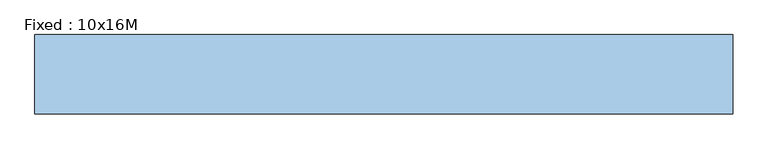
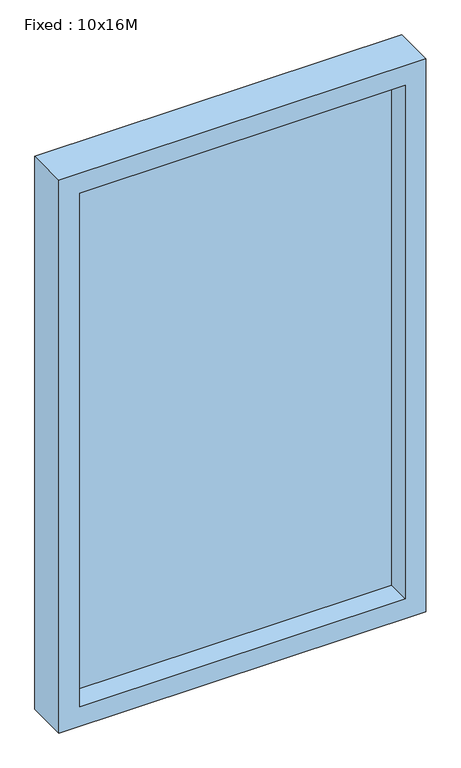
"""IFC4 building model written with IfcOpenShell, lengths in millimetres: window geometry, Fixed : 10x16M."""

from ifc_helpers import new_model, si_unit, frame, origin, place, context, project, spatial, polyline, outline, extrude, source, transform, mapped, element, save


def fixed_10x16m_885135a8(model_context):
    return source(origin(), model_context, "Body", "SweptSolid", [
        extrude(outline(polyline([(2412.0, 506.0), (2412.0, -506.0), (800.0, -506.0), (800.0, 506.0), (2412.0, 506.0)]), holes=[polyline([(857.0, 449.0), (857.0, -449.0), (2355.0, -449.0), (2355.0, 449.0), (857.0, 449.0)])]), frame((0.0, 69.0, 0.0), z_axis=(0.0, 1.0, 0.0), x_axis=(0.0, 0.0, 1.0)), (0.0, 0.0, 1.0), 115.0),
        extrude(outline(polyline([(-449.0, 162.0), (449.0, 162.0), (449.0, 134.0), (-449.0, 134.0), (-449.0, 162.0)])), frame((0.0, 0.0, 857.0), z_axis=(0.0, 0.0, 1.0), x_axis=(1.0, 0.0, 0.0)), (0.0, 0.0, 1.0), 1498.0),
    ])


if __name__ == "__main__":
    model = new_model("IFC4")
    model_context = context("Model", 3, world=origin())
    ifc_project = project(units=[si_unit("LENGTHUNIT", "METRE", prefix="MILLI")], contexts=[model_context])
    site = spatial("IfcSite", under=ifc_project)
    building = spatial("IfcBuilding", under=site)
    placement = place(None, origin())
    fixed_10x16m_shape = fixed_10x16m_885135a8(model_context)
    element("IfcWindow", 1, ObjectType="Fixed : 10x16M", at=placement, inside=building, context=model_context, shape_type="MappedRepresentation", body=[
        mapped(fixed_10x16m_shape, transform((0.0, 0.0, 0.0), x_axis=(1.0, 0.0, 0.0), y_axis=(0.0, 1.0, 0.0), z_axis=(0.0, 0.0, 1.0))),
    ])
    save(model, "model.ifc")

# Revit data of these elements
# Type "Fixed : 10x16M"
#   Type Mark = "59"
#   Creator Organization [instance default] = "© Danish Educational Content"
#   Creator Name [instance default] = "© Erik Falck Jørgensen"
#   Creator Build [instance default] = "2017.0801.0"
#   Analytic Construction = "<None>"
#   length#5 = -22 mm
#   length#4 = -50 mm
#   length#3 = 100 mm
#   length#2 = 57 mm
#   length#1 = 0 mm
#   Seal Width = 12 mm
#   Rough Width = 1012 mm
#   Rough Height = 1612 mm
#   Rebate Depth = 50 mm
#   Height = 1588 mm
#   Glass Thickness = 28 mm
#   Exterior Direction [instance default] = 0.00°
#   Default Sill Height = 800 mm
#   Width = 988 mm
#   Case Width = 45 mm
#   Case Depth = 115 mm
#   Sealing = no
#   Wall Closure = 1
#   Above Cutplane [instance default] = no
#   Wall Surface = none
#   Sill Plate = none
#   Glass = none
#   Embrasure = none
#   Case/Transom = none
#   Assembly Code = ""
# Element 1 (IfcWindow, "Fixed : 10x16M")
#   Materials on its faces: "Default Frame/Mullion (Interior/Exterior)", "Glass"
# Materials
#   "Default Frame/Mullion (Interior/Exterior)": class "Generic", colour RGB 205 205 205, transparency 0, Description = "Udefineret karm/ramme materiale", Cost = 0
#   "Glass": class "Glass", colour RGB 180 200 255, transparency 0.75, Description = "Generisk glas", Cost = 0
